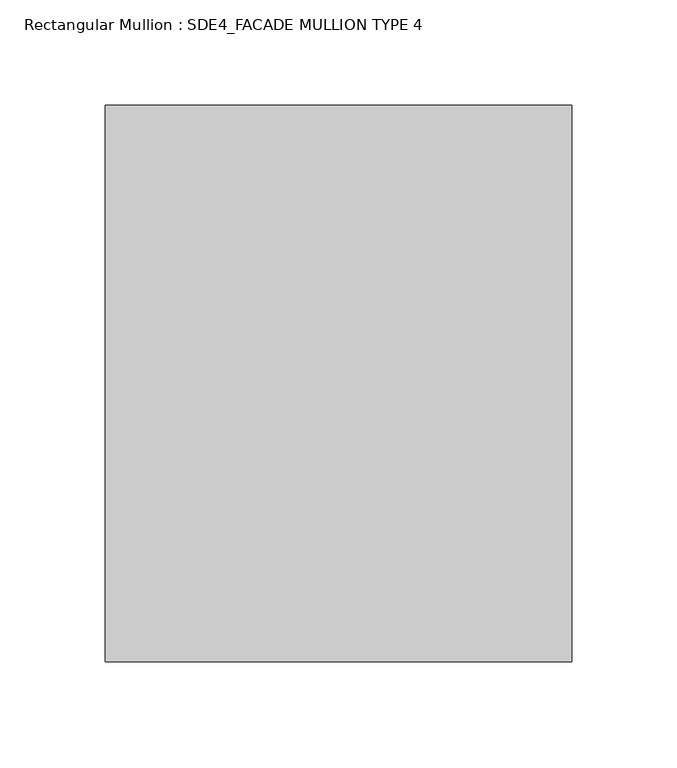
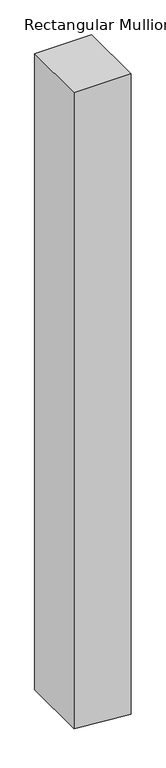
"""IFC4 building model written with IfcOpenShell, lengths in millimetres: member geometry, Rectangular Mullion : SDE4_FACADE MULLION TYPE 4."""

from ifc_helpers import new_model, si_unit, frame, origin, place, context, project, spatial, polyline, outline, extrude, source, transform, mapped, element, save


def rectangular_mullion_sde4_facade_mullion_type_4_a04de156(model_context):
    return source(origin(), model_context, "Body", "SweptSolid", [
        extrude(outline(polyline([(0.0, 111.0), (0.0, -111.0), (-2615.9425269, -111.0), (-2624.6834485, 3.056508), (-2632.9558884, 111.0), (0.0, 111.0)])), frame((0.0, -132.5, 0.0), z_axis=(0.0, 1.0, 0.0), x_axis=(0.0, 0.0, 1.0)), (0.0, 0.0, 1.0), 265.0),
    ])


if __name__ == "__main__":
    model = new_model("IFC4")
    model_context = context("Model", 3, world=origin())
    ifc_project = project(units=[si_unit("LENGTHUNIT", "METRE", prefix="MILLI")], contexts=[model_context])
    site = spatial("IfcSite", under=ifc_project)
    building = spatial("IfcBuilding", under=site)
    placement = place(None, origin())
    rectangular_mullion_sde4_facade_mullion_type_4_shape = rectangular_mullion_sde4_facade_mullion_type_4_a04de156(model_context)
    element("IfcMember", 1, ObjectType="Rectangular Mullion : SDE4_FACADE MULLION TYPE 4", at=placement, inside=building, context=model_context, shape_type="MappedRepresentation", body=[
        mapped(rectangular_mullion_sde4_facade_mullion_type_4_shape, transform((0.0, 0.0, 0.0), x_axis=(1.0, 0.0, 0.0), y_axis=(0.0, 1.0, 0.0), z_axis=(0.0, 0.0, 1.0))),
    ])
    save(model, "model.ifc")

# Revit data of these elements
# Type "Rectangular Mullion : SDE4_FACADE MULLION TYPE 4"
#   built-in parameter 1007322 = 0.869423 (stored number, unit not read)
#   built-in parameter 1007321 = 0.364173 (stored number, unit not read)
#   built-in parameter 1007320 = 0.364173 (stored number, unit not read)
